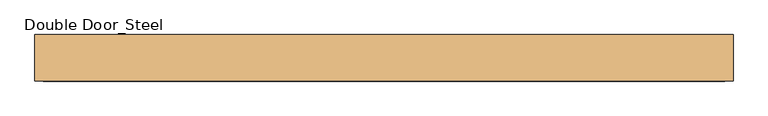
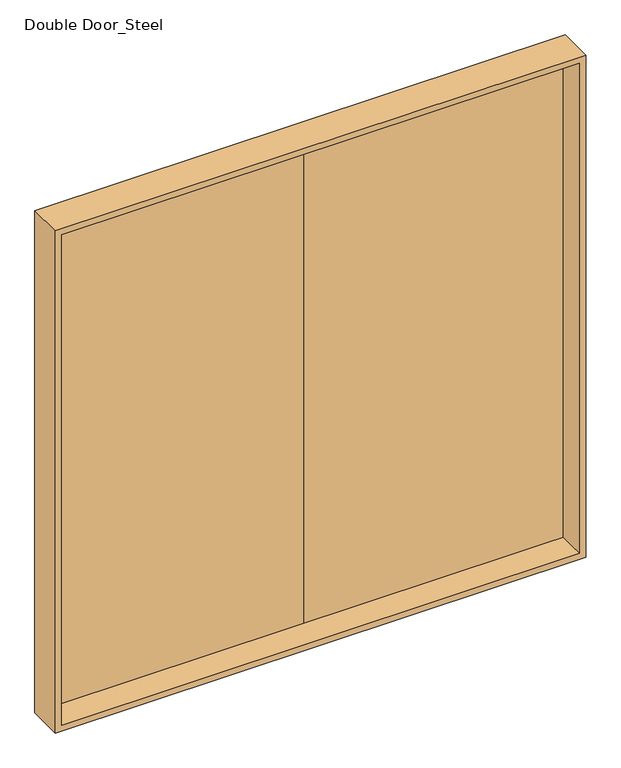
"""IFC4 building model written with IfcOpenShell, lengths in millimetres: door geometry, Double Door_Steel : H_DR_AR_B12_Double Door_Steel_W3000xH3000."""

import ifcopenshell
import ifcopenshell.guid

model = None  # the IFC model being written
_history = None  # IfcOwnerHistory: only IFC2X3 demands one
_inside = {}  # id of a spatial element -> (the spatial element, [elements in it])
_under = {}  # id of a project, library or spatial element -> (it, [spatial elements below it])
_declared = {}  # id of a project -> (the project, [libraries it declares])
_typed = {}  # id of a type object -> (the type object, [elements of that type])
_made_of = {}  # id of a material, layer set ... -> (it, [elements and type objects made of it])


def new_model(schema):
    """Start an empty IFC model of exactly this schema.

    Asked for "IFC4X3", IfcOpenShell would pick the latest addendum, in which some entities
    have other attributes; the version numbers below select the first issue.
    IFC2X3 requires an IfcOwnerHistory on every rooted entity: one is made here for all.
    """
    global model, _history
    if schema == "IFC4X3":
        model = ifcopenshell.file(schema_version=(4, 3, 0, 0))
    else:
        model = ifcopenshell.file(schema=schema)
    _inside.clear()
    _under.clear()
    _declared.clear()
    _typed.clear()
    _made_of.clear()
    _history = None
    if model.schema == "IFC2X3":
        org = make("IfcOrganization", Name="unknown")
        user = make(
            "IfcPersonAndOrganization",
            ThePerson=make("IfcPerson", FamilyName="unknown"),
            TheOrganization=org,
        )
        app = make(
            "IfcApplication",
            ApplicationDeveloper=org,
            Version="unknown",
            ApplicationFullName="unknown",
            ApplicationIdentifier="unknown",
        )
        _history = make(
            "IfcOwnerHistory",
            OwningUser=user,
            OwningApplication=app,
            ChangeAction="ADDED",
            CreationDate=0,
        )
    return model


def make(cls, **values):
    """One entity of the class cls with the attributes given. An attribute that is None is left unset."""
    return model.create_entity(
        cls, **{name: value for name, value in values.items() if value is not None}
    )


def rooted(cls, **values):
    """An entity with a GlobalId (a new one), such as an element, a storey or a relation."""
    return make(cls, GlobalId=ifcopenshell.guid.new(), OwnerHistory=_history, **values)


def si_unit(unit_type, name, prefix=None):
    """IfcSIUnit, for example si_unit("LENGTHUNIT", "METRE", prefix="MILLI")."""
    return make("IfcSIUnit", UnitType=unit_type, Prefix=prefix, Name=name)


def assignment(units):
    """IfcUnitAssignment: the units of a project."""
    return None if units is None else make("IfcUnitAssignment", Units=units)


def point(xyz):
    """IfcCartesianPoint."""
    return None if xyz is None else make("IfcCartesianPoint", Coordinates=xyz)


def direction(xyz):
    """IfcDirection."""
    return None if xyz is None else make("IfcDirection", DirectionRatios=xyz)


def frame(location, z_axis=None, x_axis=None):
    """IfcAxis2Placement3D, a coordinate frame: its origin and axes. An axis left out is left unset."""
    return make(
        "IfcAxis2Placement3D",
        Location=point(location),
        Axis=direction(z_axis),
        RefDirection=direction(x_axis),
    )


def origin():
    """The frame at (0, 0, 0) with its axes left unset."""
    return frame((0.0, 0.0, 0.0))


def place(relative_to, where):
    """IfcLocalPlacement: puts the frame where relative to a parent placement (None: the world)."""
    return make(
        "IfcLocalPlacement", PlacementRelTo=relative_to, RelativePlacement=where
    )


def context(
    kind, dimensions, precision=None, world=None, true_north=None, identifier=None
):
    """IfcGeometricRepresentationContext, for example the 3D "Model" context."""
    return make(
        "IfcGeometricRepresentationContext",
        ContextIdentifier=identifier,
        ContextType=kind,
        CoordinateSpaceDimension=dimensions,
        Precision=precision,
        WorldCoordinateSystem=world,
        TrueNorth=true_north,
    )


def project(units=None, contexts=None):
    """IfcProject with its units and contexts."""
    return rooted(
        "IfcProject",
        Name="project",
        RepresentationContexts=contexts,
        UnitsInContext=assignment(units),
    )


def spatial(cls, under=None, at=None, **own):
    """A site, building, storey or space (cls), placed at a placement, below another one or the project."""
    s = rooted(cls, ObjectPlacement=at, **own)
    if under is not None:
        _under.setdefault(under.id(), (under, []))[1].append(s)
    return s


def polyline(points):
    """IfcPolyline through the points."""
    return make("IfcPolyline", Points=[point(p) for p in points])


def outline(outer, holes=None, kind="AREA"):
    """IfcArbitraryClosedProfileDef: a profile drawn as a closed curve; with holes, ...WithVoids."""
    if holes is None:
        return make("IfcArbitraryClosedProfileDef", ProfileType=kind, OuterCurve=outer)
    return make(
        "IfcArbitraryProfileDefWithVoids",
        ProfileType=kind,
        OuterCurve=outer,
        InnerCurves=holes,
    )


def extrude(swept, where, along, depth):
    """IfcExtrudedAreaSolid: the profile swept, set in the frame where, extruded along a direction by depth."""
    return make(
        "IfcExtrudedAreaSolid",
        SweptArea=swept,
        Position=where,
        ExtrudedDirection=direction(along),
        Depth=depth,
    )


def faces_of(points, faces, orient=None, outer=None):
    """IfcFace entities. A face is a list of loops; a loop is a list of indices into points, from 0.

    orient and outer hold one flag for each loop. By default every Orientation is true, the
    first loop of a face is its IfcFaceOuterBound and the others are IfcFaceBound.
    """
    made = []
    for i, loops in enumerate(faces):
        bounds = []
        for j, loop in enumerate(loops):
            is_outer = j == 0 if outer is None else outer[i][j]
            bounds.append(
                make(
                    "IfcFaceOuterBound" if is_outer else "IfcFaceBound",
                    Bound=make("IfcPolyLoop", Polygon=[points[k] for k in loop]),
                    Orientation=True if orient is None else orient[i][j],
                )
            )
        made.append(make("IfcFace", Bounds=bounds))
    return made


def faceted_brep(points, faces, orient=None, outer=None, voids=None):
    """IfcFacetedBrep: a solid bounded by flat faces; with voids (closed shells), ...WithVoids."""
    shared = [point(p) for p in points]
    hull = make("IfcClosedShell", CfsFaces=faces_of(shared, faces, orient, outer))
    if voids is None:
        return make("IfcFacetedBrep", Outer=hull)
    return make(
        "IfcFacetedBrepWithVoids",
        Outer=hull,
        Voids=[
            make(cls, CfsFaces=faces_of(shared, fs, o, b)) for cls, fs, o, b in voids
        ],
    )


def shape(context_of_items, identifier, shape_type, items):
    """IfcShapeRepresentation: the items that make up one representation, for example the "Body"."""
    return make(
        "IfcShapeRepresentation",
        ContextOfItems=context_of_items,
        RepresentationIdentifier=identifier,
        RepresentationType=shape_type,
        Items=items,
    )


def source(mapping_origin, context_of_items, identifier, shape_type, items):
    """IfcRepresentationMap: a shape defined once, which mapped items show again and again."""
    return make(
        "IfcRepresentationMap",
        MappingOrigin=mapping_origin,
        MappedRepresentation=shape(context_of_items, identifier, shape_type, items),
    )


def transform(
    local_origin,
    x_axis=None,
    y_axis=None,
    z_axis=None,
    scale=None,
    scale2=None,
    scale3=None,
    uniform=True,
):
    """IfcCartesianTransformationOperator3D, or its non-uniform kind. x_axis, y_axis, z_axis: its Axis1, 2, 3."""
    if uniform:
        return make(
            "IfcCartesianTransformationOperator3D",
            Axis1=direction(x_axis),
            Axis2=direction(y_axis),
            LocalOrigin=point(local_origin),
            Scale=scale,
            Axis3=direction(z_axis),
        )
    return make(
        "IfcCartesianTransformationOperator3DnonUniform",
        Axis1=direction(x_axis),
        Axis2=direction(y_axis),
        LocalOrigin=point(local_origin),
        Scale=scale,
        Axis3=direction(z_axis),
        Scale2=scale2,
        Scale3=scale3,
    )


def mapped(mapping_source, mapping_target):
    """IfcMappedItem: shows the shape of a source again, moved by a transform."""
    return make(
        "IfcMappedItem", MappingSource=mapping_source, MappingTarget=mapping_target
    )


def made_of(thing, what):
    """Note that an element or type object is made of a material, layer set ...; save() writes the relation."""
    if what is not None:
        _made_of.setdefault(what.id(), (what, []))[1].append(thing)
    return thing


def element(
    cls,
    number,
    at=None,
    inside=None,
    cuts=None,
    type_object=None,
    material=None,
    context=None,
    identifier="Body",
    shape_type=None,
    held_by="IfcProductDefinitionShape",
    body=None,
    shapes=None,
    **own,
):
    """One element of the class cls, such as IfcWall. Its Tag is "e" and its number.

    at: its placement. inside: the storey or other place that contains it. cuts: it is an
    opening in that element (IfcRelVoidsElement). A single representation is given by context,
    identifier, shape_type and body (its items); several are given by shapes. held_by: the class
    of the entity that holds the representations. save() writes the other relations.
    """
    e = rooted(cls, Tag="e%d" % number, ObjectPlacement=at, **own)
    if body is not None:
        shapes = [shape(context, identifier, shape_type, body)]
    if shapes is not None:
        e.Representation = make(held_by, Representations=shapes)
    if inside is not None:
        _inside.setdefault(inside.id(), (inside, []))[1].append(e)
    if cuts is not None:
        rooted(
            "IfcRelVoidsElement", RelatingBuildingElement=cuts, RelatedOpeningElement=e
        )
    if type_object is not None:
        _typed.setdefault(type_object.id(), (type_object, []))[1].append(e)
    return made_of(e, material)


def aggregate(whole, parts):
    """IfcRelAggregates: a whole, such as a stair, and the parts it consists of."""
    return rooted("IfcRelAggregates", RelatingObject=whole, RelatedObjects=parts)


def save(model, path):
    """Write the relations noted so far, then the file.

    IfcRelAggregates (storeys below a building ...), IfcRelContainedInSpatialStructure (elements
    in a storey), IfcRelDefinesByType, IfcRelAssociatesMaterial and IfcRelDeclares: one each for
    every whole, place, type object, material and project.
    """
    for whole, parts in _under.values():
        aggregate(whole, parts)
    for where, things in _inside.values():
        rooted(
            "IfcRelContainedInSpatialStructure",
            RelatedElements=things,
            RelatingStructure=where,
        )
    for kind, things in _typed.values():
        rooted("IfcRelDefinesByType", RelatedObjects=things, RelatingType=kind)
    for what, things in _made_of.values():
        rooted("IfcRelAssociatesMaterial", RelatedObjects=things, RelatingMaterial=what)
    for by, libraries in _declared.values():
        rooted("IfcRelDeclares", RelatingContext=by, RelatedDefinitions=libraries)
    model.write(path)


def double_door_steel_ab4802d0(model_context):
    return source(origin(), model_context, "Body", "SolidModel", [
        extrude(outline(polyline([(1480.0, 60.0), (0.0, 60.0), (0.0, 100.0), (1480.0, 100.0), (1480.0, 60.0)])), frame((0.0, 0.0, 20.0), z_axis=(0.0, 0.0, 1.0), x_axis=(1.0, 0.0, 0.0)), (0.0, 0.0, 1.0), 2960.0),
        extrude(outline(polyline([(0.0, 60.0), (-1480.0, 60.0), (-1480.0, 100.0), (0.0, 100.0), (0.0, 60.0)])), frame((0.0, 0.0, 20.0), z_axis=(0.0, 0.0, 1.0), x_axis=(1.0, 0.0, 0.0)), (0.0, 0.0, 1.0), 2960.0),
        faceted_brep([(1500.0, -100.0, 3000.0), (1500.0, 100.0, 3000.0), (-1500.0, 100.0, 3000.0), (-1500.0, -100.0, 3000.0), (1465.0, 60.0, 2965.0), (1465.0, -100.0, 2965.0), (-1465.0, -100.0, 2965.0), (-1465.0, 60.0, 2965.0), (1480.0, 100.0, 2980.0), (1480.0, 60.0, 2980.0), (-1480.0, 60.0, 2980.0), (-1480.0, 100.0, 2980.0), (-1500.0, 100.0, 0.0), (-1500.0, -100.0, 0.0), (-1465.0, -100.0, 35.0), (-1465.0, 60.0, 35.0), (-1480.0, 60.0, 20.0), (-1480.0, 100.0, 20.0), (1500.0, 100.0, 0.0), (1480.0, 100.0, 20.0), (1500.0, -100.0, 0.0), (1465.0, -100.0, 35.0), (1465.0, 60.0, 35.0), (1480.0, 60.0, 20.0)], [[[0, 1, 2, 3]], [[4, 5, 6, 7]], [[8, 9, 10, 11]], [[3, 2, 12, 13]], [[7, 6, 14, 15]], [[11, 10, 16, 17]], [[18, 12, 2, 1], [8, 11, 17, 19]], [[13, 12, 18, 20]], [[0, 3, 13, 20], [21, 14, 6, 5]], [[15, 14, 21, 22]], [[23, 16, 10, 9], [4, 7, 15, 22]], [[17, 16, 23, 19]], [[20, 18, 1, 0]], [[22, 21, 5, 4]], [[19, 23, 9, 8]]]),
    ])


if __name__ == "__main__":
    model = new_model("IFC4")
    model_context = context("Model", 3, world=origin())
    ifc_project = project(units=[si_unit("LENGTHUNIT", "METRE", prefix="MILLI")], contexts=[model_context])
    site = spatial("IfcSite", under=ifc_project)
    building = spatial("IfcBuilding", under=site)
    placement = place(None, origin())
    double_door_steel_shape = double_door_steel_ab4802d0(model_context)
    element("IfcDoor", 1, ObjectType="Double Door_Steel : H_DR_AR_B12_Double Door_Steel_W3000xH3000", at=placement, inside=building, context=model_context, shape_type="MappedRepresentation", body=[
        mapped(double_door_steel_shape, transform((0.0, 0.0, 0.0), x_axis=(1.0, 0.0, 0.0), y_axis=(0.0, 1.0, 0.0), z_axis=(0.0, 0.0, 1.0))),
    ])
    save(model, "model.ifc")

# Revit data of these elements
# Type "Double Door_Steel : H_DR_AR_B12_Double Door_Steel_W3000xH3000"
#   Type Mark = "430"
#   프레임 = ""
#   철물 = ""
#   유리/마감 = ""
#   위치/개소 = ""
#   부호 = "1/SD"
#   문번호 = ""
#   문기호 = "SD"
#   Analytic Construction = "<None>"
#   Height = 3000 mm
#   Width = 3000 mm
#   Define Thermal Properties by = 1
#   문 틀 = none
#   문 = none
#   Function = (empty or 0)
#   Assembly Code = ""
#   Wall Closure = (empty or 0)
